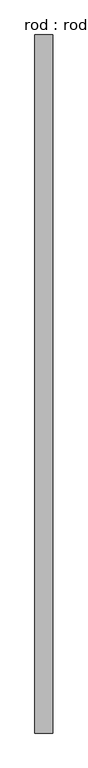
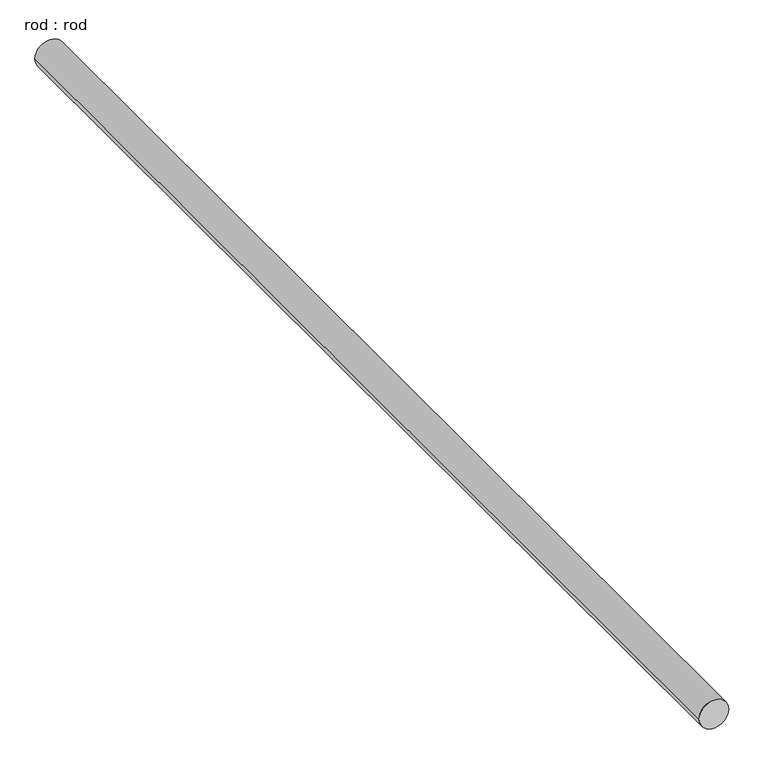
"""IFC4 building model written with IfcOpenShell, lengths in millimetres: proxy geometry, rod : rod."""

from ifc_helpers import new_model, si_unit, point, frame, frame_2d, origin, place, context, project, spatial, circle_curve, trimmed, segment, composite_curve, outline, extrude, source, transform, mapped, element, save


def rod_rod_699355d6(model_context):
    return source(origin(), model_context, "Body", "SweptSolid", [
        extrude(outline(composite_curve([segment(trimmed(circle_curve(frame_2d((0.0108462, 0.0)), 200.0), [point((0.0108462, 200.0))], [point((0.0108462, -200.0))], False, "CARTESIAN"), True, "CONTINUOUS"), segment(trimmed(circle_curve(frame_2d((0.0108462, 0.0)), 200.0), [point((0.0108462, -200.0))], [point((0.0108462, 200.0))], False, "CARTESIAN"), True, "CONTINUOUS")], self_intersect=False)), frame((0.0, -3657.2713847, 0.0), z_axis=(0.0, 1.0, 0.0), x_axis=(0.0, 0.0, 1.0)), (0.0, 0.0, 1.0), 15500.0),
    ])


if __name__ == "__main__":
    model = new_model("IFC4")
    model_context = context("Model", 3, world=origin())
    ifc_project = project(units=[si_unit("LENGTHUNIT", "METRE", prefix="MILLI")], contexts=[model_context])
    site = spatial("IfcSite", under=ifc_project)
    building = spatial("IfcBuilding", under=site)
    placement = place(None, origin())
    rod_rod_shape = rod_rod_699355d6(model_context)
    element("IfcBuildingElementProxy", 1, Name="rod : rod", ObjectType="rod : rod", at=placement, inside=building, context=model_context, shape_type="MappedRepresentation", body=[
        mapped(rod_rod_shape, transform((0.0, 0.0, 0.0), x_axis=(1.0, 0.0, 0.0), y_axis=(0.0, 1.0, 0.0), z_axis=(0.0, 0.0, 1.0))),
    ])
    save(model, "model.ifc")

# Revit data of these elements
# Type "rod : rod"
#   Default Elevation = 0
